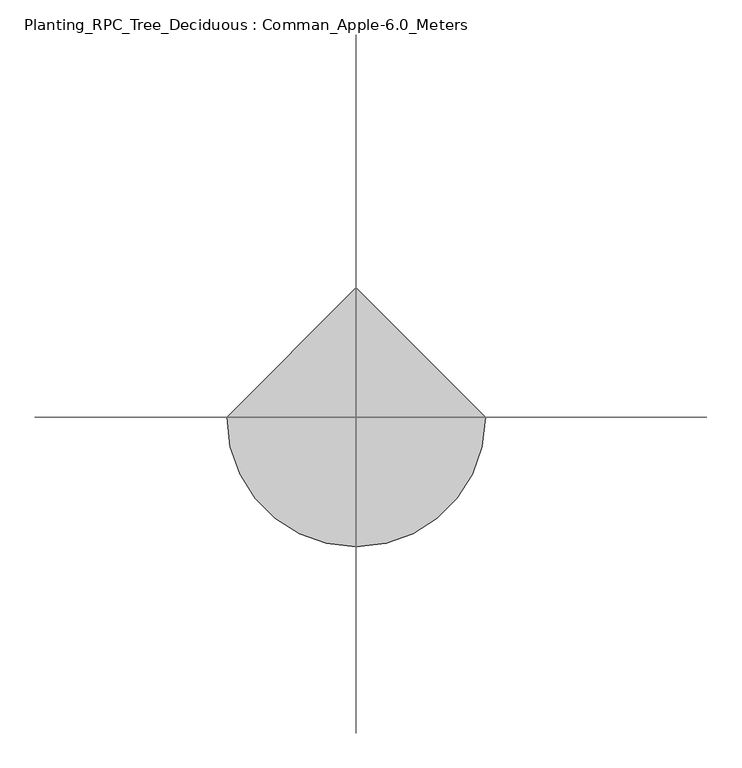
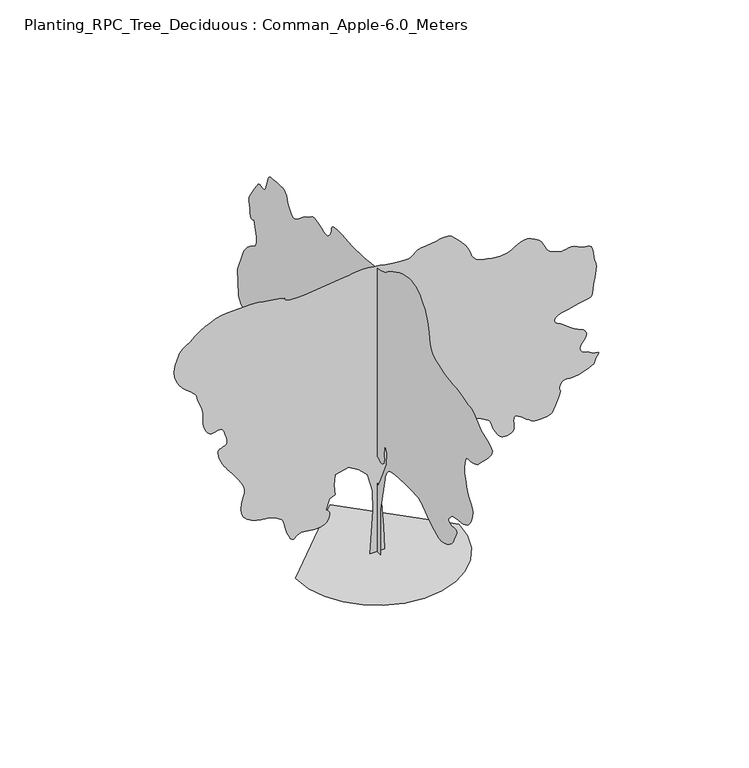
"""IFC4 building model written with IfcOpenShell, lengths in millimetres: geographic element geometry, Planting_RPC_Tree_Deciduous : Comman_Apple-6.0_Meters."""

from ifc_helpers import new_model, si_unit, origin, place, context, project, spatial, triangles, source, transform, mapped, element, save


def planting_rpc_tree_deciduous_comman_apple_6_0_meters_31fc5fb8(model_context):
    return source(origin(), model_context, "Body", "Tessellation", [
        triangles([(-6.51e-05, -105.0228319, 0.0074776), (-6.15e-05, 138.9131143, 0.0074703), (-4.84e-05, 99.8833291, 458.6078719), (-3.14e-05, 129.1556067, 1014.7807915), (-1.8e-05, 226.7299288, 1414.8361691), (-8.5e-06, 392.6053236, 1649.0138809), (-1.1e-06, 577.9979682, 1805.1340027), (2.6e-06, 753.6305981, 1844.161417), (3.5e-06, 948.7807503, 1775.8613708), (1.5e-06, 1007.3257959, 1678.2863674), (-4e-06, 890.2357046, 1551.4387321), (-8.4e-06, 929.2657351, 1385.5636826), (-1.44e-05, 1153.685903, 1073.3258371), (-1.47e-05, 1543.9838093, 868.4182137), (-8.5e-06, 2109.9142365, 790.3606236), (7.6e-06, 2451.4244957, 1161.1409712), (2.53e-05, 2802.702182, 1580.7112186), (3.2e-05, 3349.1028419, 1531.9237896), (3.84e-05, 3544.2528488, 1649.0138809), (4.53e-05, 3534.5028625, 1883.1915928), (4.5e-05, 3358.8778267, 1961.2516537), (4.95e-05, 3232.0277206, 2175.9142776), (5.43e-05, 3534.5028625, 2185.6718216), (5.98e-05, 4139.453437, 2068.584201), (6.19e-05, 4208.0283211, 2104.1717091), (6.39e-05, 4273.9283684, 2140.0142887), (6.59e-05, 4334.553447, 2176.3691917), (6.78e-05, 4387.2284294, 2213.4942513), (6.96e-05, 4429.328476, 2251.6417774), (7.12e-05, 4458.2034576, 2291.0693127), (7.26e-05, 4471.2035362, 2332.0343994), (8.79e-05, 4500.4784935, 2829.6522812), (9.79e-05, 4334.6034439, 3249.2275429), (9.86e-05, 4317.5036156, 3282.3275574), (9.94e-05, 4292.2284142, 3321.5527794), (0.0001002, 4260.1033401, 3364.7027618), (0.000101, 4222.5283081, 3409.5526405), (0.0001017, 4180.8532356, 3453.9028404), (0.0001023, 4136.4533295, 3495.527916), (0.0001027, 4090.6782166, 3532.2027122), (0.0001029, 4046.5782921, 3560.9279938), (0.0001029, 4006.7531067, 3582.8278198), (0.000103, 3971.8782005, 3601.8278229), (0.0001031, 3942.6282417, 3621.853054), (0.0001036, 3919.7031876, 3646.8529816), (0.0001043, 3903.7782875, 3680.7029503), (0.0001056, 3895.5282097, 3727.3530098), (0.0001072, 3894.4782738, 3782.2781456), (0.0001089, 3899.0532852, 3838.2282188), (0.0001108, 3908.3283005, 3895.0532387), (0.0001127, 3921.3530869, 3952.5282188), (0.0001147, 3937.2032822, 4010.528167), (0.0001167, 3954.9280724, 4068.8783844), (0.0001187, 3973.5780968, 4127.4033005), (0.0001184, 3998.5533165, 4107.2783661), (0.0001184, 4022.8532867, 4091.9534294), (0.0001185, 4045.7783409, 4086.1782005), (0.0001191, 4066.6532295, 4094.7532585), (0.0001202, 4084.8032845, 4122.4283134), (0.0001219, 4099.5532562, 4174.003363), (0.0001245, 4110.1781891, 4254.2534065), (0.000127, 4120.6784203, 4333.2285278), (0.0001287, 4132.0283089, 4385.4035408), (0.0001299, 4139.1284569, 4422.2036201), (0.0001309, 4136.8033081, 4455.0786484), (0.0001318, 4120.0034615, 4495.478508), (0.0001331, 4083.5533607, 4554.8286644), (0.0001348, 4022.3783157, 4644.5537109), (0.0001367, 3956.5782623, 4741.1289207), (0.0001382, 3906.9780922, 4815.003772), (0.0001392, 3869.5280525, 4868.5789902), (0.0001398, 3840.0781059, 4904.2041412), (0.0001401, 3814.5532104, 4924.3290756), (0.0001399, 3788.8780334, 4931.3042313), (0.0001393, 3758.9281174, 4927.5038818), (0.0001386, 3727.67799, 4918.0288788), (0.0001379, 3700.2029228, 4909.0788437), (0.0001374, 3675.45298, 4904.7291092), (0.0001372, 3652.4029335, 4909.0788437), (0.0001374, 3630.0528442, 4926.2289597), (0.000138, 3607.3527763, 4960.2792068), (0.0001393, 3583.2777924, 5015.329335), (0.0001409, 3562.2279144, 5079.6288986), (0.0001424, 3546.3027237, 5137.7544205), (0.0001437, 3531.0527824, 5188.4042358), (0.0001447, 3512.0527794, 5230.1540131), (0.0001452, 3484.8526955, 5261.6794144), (0.0001452, 3445.0278008, 5281.604361), (0.0001446, 3388.1277855, 5288.5295197), (0.0001436, 3319.3276245, 5291.5793335), (0.0001428, 3248.6275795, 5298.5544891), (0.000142, 3178.9774704, 5306.2040222), (0.0001411, 3113.2274139, 5311.3042923), (0.0001402, 3054.3025223, 5310.5793365), (0.0001392, 3005.1273262, 5300.8293503), (0.000138, 2968.5775223, 5278.7795334), (0.0001369, 2944.7272339, 5253.1543533), (0.0001361, 2929.602285, 5232.6294434), (0.0001354, 2919.9272942, 5214.0044174), (0.0001347, 2912.4774582, 5194.0044754), (0.0001338, 2904.0023941, 5169.4042328), (0.0001326, 2891.2523003, 5136.9288895), (0.000131, 2871.0023735, 5093.3792221), (0.0001292, 2844.6522377, 5045.379245), (0.0001275, 2815.5772682, 5003.1539154), (0.000126, 2783.4271957, 4968.9542587), (0.0001248, 2747.8773308, 4945.0039764), (0.0001238, 2708.5521149, 4933.504097), (0.0001233, 2665.1521477, 4936.7039017), (0.0001232, 2617.3021614, 4956.7788391), (0.0001234, 2569.6771614, 4988.2542435), (0.0001238, 2525.4769524, 5023.3038483), (0.0001243, 2482.1194244, 5060.7288895), (0.0001247, 2437.0595295, 5099.3538574), (0.0001252, 2387.7318718, 5138.0044052), (0.0001254, 2331.5768692, 5175.4294464), (0.0001255, 2266.0343582, 5210.4790512), (0.0001256, 2205.0142456, 5244.5542969), (0.0001259, 2159.0142918, 5277.6040237), (0.0001262, 2120.3541515, 5306.2290207), (0.0001262, 2081.3542065, 5327.0044968), (0.0001258, 2034.3291698, 5336.5044983), (0.0001247, 1971.6040741, 5331.3292328), (0.0001227, 1885.4940685, 5308.0544907), (0.0001205, 1797.391452, 5276.8540695), (0.0001188, 1730.2863911, 5251.9544266), (0.0001175, 1678.8813892, 5236.1042313), (0.0001168, 1637.8888332, 5232.02948), (0.0001166, 1602.0163136, 5242.4794235), (0.0001169, 1565.9737461, 5270.1544785), (0.0001177, 1524.4687214, 5317.8044769), (0.0001188, 1490.9861721, 5373.8045471), (0.0001201, 1475.2561729, 5423.9793915), (0.0001212, 1466.3511932, 5467.3296524), (0.0001221, 1453.3511147, 5502.8292297), (0.0001225, 1425.3286972, 5529.4543488), (0.0001222, 1371.366148, 5546.1794907), (0.000121, 1280.5334656, 5551.979718), (0.0001195, 1182.4759335, 5550.8792038), (0.0001183, 1108.9958982, 5547.8793869), (0.0001174, 1052.4133781, 5543.5296524), (0.0001165, 1005.0483187, 5538.3293884), (0.0001156, 959.2208107, 5532.7797272), (0.0001147, 907.2482563, 5527.4044739), (0.0001136, 841.4482029, 5522.7041794), (0.0001125, 772.3506037, 5519.7043625), (0.0001115, 711.6155754, 5518.9044113), (0.0001107, 653.2705175, 5520.154335), (0.0001099, 591.3404677, 5523.2797256), (0.000109, 519.8504273, 5528.1294296), (0.0001078, 432.8303392, 5534.5046219), (0.0001065, 324.3052774, 5542.2297318), (0.000105, 203.687658, 5552.8796631), (0.0001037, 86.9965703, 5567.6043457), (0.0001026, -21.8426915, 5585.7544006), (0.0001018, -118.9050968, 5606.6292892), (0.0001012, -200.2644113, 5629.5546341), (0.0001011, -261.9952181, 5653.8543137), (0.0001012, -300.1702499, 5678.8295334), (0.0001016, -342.4727732, 5713.0297714), (0.000102, -413.9603428, 5761.2297363), (0.0001023, -506.7854181, 5817.0798157), (0.0001024, -613.0930281, 5874.3298096), (0.0001023, -725.0330704, 5926.6045258), (0.0001019, -834.75319, 5967.6299286), (0.0001011, -934.4057556, 5991.07966), (0.0001, -1022.9033335, 5999.8047089), (9.88e-05, -1104.7484104, 6000.0046967), (9.74e-05, -1180.4459702, 5990.3047073), (9.57e-05, -1250.5110249, 5969.3298248), (9.38e-05, -1315.4560432, 5935.7295502), (9.14e-05, -1375.7936394, 5888.1545471), (8.87e-05, -1432.0336658, 5825.2049011), (8.63e-05, -1478.7161362, 5768.8048553), (8.48e-05, -1512.7687088, 5733.7546692), (8.36e-05, -1538.2837212, 5707.9295013), (8.25e-05, -1559.3638298, 5679.2045105), (8.09e-05, -1580.1012268, 5635.454274), (7.84e-05, -1604.5962433, 5564.5545319), (7.46e-05, -1636.941362, 5454.4042786), (7.05e-05, -1667.1512913, 5330.3292938), (6.7e-05, -1688.656374, 5223.97939), (6.39e-05, -1710.6739254, 5132.8541382), (6.11e-05, -1742.4214062, 5054.3292801), (5.83e-05, -1793.1164223, 4985.8788071), (5.53e-05, -1871.9714928, 4924.9540375), (5.19e-05, -1988.2065491, 4868.9789658), (4.87e-05, -2119.0091755, 4825.5040031), (4.62e-05, -2237.6917568, 4799.6038399), (4.41e-05, -2347.6668755, 4784.9788605), (4.22e-05, -2452.3543808, 4775.3288681), (4.04e-05, -2555.1521759, 4764.2789612), (3.83e-05, -2659.5022018, 4745.5539413), (3.57e-05, -2768.8022163, 4712.8539024), (3.33e-05, -2866.4523605, 4683.5786545), (3.19e-05, -2939.5522591, 4672.2287659), (3.09e-05, -2996.927536, 4668.05373), (2.99e-05, -3047.4773575, 4660.2786232), (2.85e-05, -3100.0776352, 4638.1788094), (2.61e-05, -3163.6025368, 4590.9787834), (2.24e-05, -3246.9276833, 4507.9536186), (1.83e-05, -3354.9527756, 4422.0536293), (1.48e-05, -3474.4277504, 4364.5036537), (1.18e-05, -3586.9278603, 4321.8033531), (9.3e-06, -3673.9780701, 4280.47855), (7e-06, -3717.153051, 4227.0283241), (5e-06, -3698.0280556, 4147.9782074), (2.9e-06, -3598.1780457, 4029.8281517), (1.1e-06, -3473.4528099, 3906.2781349), (-3e-07, -3385.2276718, 3815.6781418), (-1.3e-06, -3323.4776619, 3751.5279877), (-1.9e-06, -3278.1025246, 3707.3530678), (-2.2e-06, -3239.0275841, 3676.6529068), (-2.3e-06, -3196.2275803, 3652.9528999), (-2.1e-06, -3139.5775497, 3629.777861), (-1.7e-06, -3075.1774109, 3613.37799), (-9e-07, -3016.2275208, 3608.6029907), (-2e-07, -2963.4272552, 3606.7278145), (2e-07, -2917.4774437, 3599.0529922), (2e-07, -2879.0024666, 3576.8528938), (-7e-07, -2848.7272797, 3531.452758), (-2.7e-06, -2827.3524216, 3454.1278267), (-5.1e-06, -2815.7522575, 3369.9277336), (-7e-06, -2813.352404, 3305.0276253), (-8.6e-06, -2818.6523712, 3252.4026398), (-1.02e-05, -2830.0772552, 3205.052623), (-1.19e-05, -2846.1274384, 3156.0024193), (-1.39e-05, -2865.2274353, 3098.2524559), (-1.64e-05, -2885.9023361, 3024.8025787), (-1.92e-05, -2914.627327, 2946.6774055), (-2.18e-05, -2954.4525124, 2877.5772629), (-2.43e-05, -2998.5524368, 2814.6273262), (-2.67e-05, -3040.0775185, 2754.9021927), (-2.9e-05, -3072.2275909, 2695.5270378), (-3.11e-05, -3088.152491, 2633.6020386), (-3.3e-05, -3081.0526337, 2566.2020828), (-3.46e-05, -3060.4274391, 2500.277037), (-3.6e-05, -3039.102578, 2443.7194427), (-3.71e-05, -3015.2525803, 2395.18694), (-3.79e-05, -2986.9272743, 2353.3118797), (-3.85e-05, -2952.3273514, 2316.7293743), (-3.88e-05, -2909.5023491, 2284.0717747), (-3.89e-05, -2856.6273788, 2253.9743385), (-3.87e-05, -2791.7272705, 2230.5618141), (-3.8e-05, -2717.452153, 2216.0268002), (-3.71e-05, -2638.7520149, 2206.0967377), (-3.62e-05, -2560.5271385, 2196.5117123), (-3.56e-05, -2487.799601, 2182.9993103), (-3.53e-05, -2425.47201, 2161.2942398), (-3.56e-05, -2378.5043827, 2127.129174), (-3.62e-05, -2345.7043499, 2089.8041267), (-3.68e-05, -2322.8044395, 2060.3341232), (-3.73e-05, -2310.1443111, 2037.0066227), (-3.78e-05, -2308.0692924, 2018.1191128), (-3.84e-05, -2316.9168629, 2001.9616688), (-3.92e-05, -2337.0294434, 1986.8265461), (-4.01e-05, -2368.7469841, 1971.0090523), (-4.1e-05, -2411.2470062, 1962.5040482), (-4.16e-05, -2459.0394379, 1965.0915356), (-4.21e-05, -2505.4770103, 1970.754126), (-4.27e-05, -2543.876992, 1971.4641117), (-4.34e-05, -2567.6019974, 1959.2041042), (-4.44e-05, -2569.9771431, 1925.949012), (-4.59e-05, -2544.3769615, 1863.6765049), (-4.75e-05, -2509.7520401, 1792.5014889), (-4.89e-05, -2484.8695473, 1735.1513557), (-4.99e-05, -2462.7095627, 1687.5312973), (-5.08e-05, -2436.2819607, 1645.5438892), (-5.14e-05, -2398.5894939, 1605.0912712), (-5.19e-05, -2342.631863, 1562.0787804), (-5.22e-05, -2261.4142914, 1512.4087017), (-5.2e-05, -2169.1316975, 1473.3237328), (-5.1e-05, -2083.5066914, 1461.3762062), (-4.95e-05, -2002.8290577, 1471.4462311), (-4.76e-05, -1925.3965748, 1498.4137711), (-4.53e-05, -1849.4990273, 1537.1587898), (-4.28e-05, -1773.4289612, 1582.5612511), (-4.02e-05, -1695.4838642, 1629.498793), (-3.77e-05, -1622.0063725, 1676.8063705), (-3.54e-05, -1558.0838207, 1724.7964645), (-3.31e-05, -1500.136195, 1770.5689613), (-3.11e-05, -1444.578685, 1811.2214218), (-2.93e-05, -1387.8261898, 1843.8489361), (-2.77e-05, -1326.2960793, 1865.5564774), (-2.64e-05, -1256.4010723, 1873.4340488), (-2.5e-05, -1159.1384045, 1874.2890839), (-2.3e-05, -1027.910804, 1875.4840691), (-2.07e-05, -877.7382116, 1874.971455), (-1.86e-05, -723.6380974, 1870.7039829), (-1.67e-05, -580.6329818, 1860.6339581), (-1.55e-05, -463.7428782, 1842.7115055), (-1.52e-05, -387.9878002, 1814.8914013), (-1.57e-05, -343.2127716, 1776.8839828), (-1.66e-05, -308.1652379, 1730.6863667), (-1.77e-05, -281.2252217, 1677.6614056), (-1.92e-05, -260.7727092, 1619.1738419), (-2.08e-05, -245.1829449, 1556.5887085), (-2.26e-05, -232.8366963, 1491.2736546), (-2.44e-05, -222.1121874, 1424.593713), (-3.85e-05, -114.7803395, 897.6907001), (-2.01e-05, -26.9632729, 1297.7460777), (-1.3e-05, -173.3248856, 1609.9838505), (-6.5e-06, -300.1727388, 1892.9489914), (2e-07, -319.6852469, 2127.129174), (4.7e-06, -251.3852008, 2244.2167946), (-4e-07, -222.1119331, 2058.8266571), (-1.7e-06, -228.0859325, 2017.1791992), (-3e-06, -232.2679447, 1976.5565334), (-4.1e-06, -232.865183, 1937.9815624), (-5.1e-06, -228.0859325, 1902.4790783), (-5.9e-06, -216.1379336, 1871.0740185), (-6.4e-06, -195.2293988, 1844.788995), (-6.5e-06, -163.5673779, 1824.6489452), (-6.1e-06, -127.1833524, 1819.4714996), (-5.2e-06, -93.5303284, 1831.0190506), (-4.2e-06, -62.949051, 1849.7389835), (-3.3e-06, -35.7820297, 1866.0664753), (-2.9e-06, -12.3698845, 1870.4490566), (-3.1e-06, 6.9458055, 1853.3239391), (-4.3e-06, 21.8237678, 1805.1340027), (-6.1e-06, 32.3777771, 1741.0688725), (-7.7e-06, 39.3472803, 1682.1263947), (-9.3e-06, 43.330036, 1627.4512436), (-1.08e-05, 44.9230347, 1576.1888203), (-1.22e-05, 44.724037, 1527.4862698), (-1.37e-05, 43.330036, 1480.4911732), (-1.51e-05, 41.3385332, 1434.3511116), (137.391859, 0.0003253, 0.0), (-133.3141101, 0.0003334, 0.0), (-73.1573078, 0.0002372, 832.1731876), (-83.1833128, 0.0002433, 1223.1935062), (-183.4456522, 0.0001982, 1574.1087147), (-333.8377625, 0.0002049, 1724.5014244), (-534.3604428, 0.0002126, 1844.8164642), (-785.015601, 0.0002192, 1784.6589443), (-805.0681561, 0.0002168, 1584.1363003), (-785.015601, 0.0002134, 1393.6386257), (-885.278231, 0.0002156, 1343.5060753), (-955.4607931, 0.0002149, 1153.0084007), (-936.3432827, 0.0002675, 1139.8859459), (-918.5407356, 0.0002668, 1125.3558735), (-903.3707314, 0.0002661, 1108.0234285), (-892.1456898, 0.0002654, 1086.4808481), (-886.1831903, 0.0002648, 1059.3258196), (-886.7981964, 0.0002643, 1025.1533415), (-895.3032005, 0.0002639, 982.5658247), (-913.9532249, 0.0002639, 940.0632591), (-942.5982788, 0.0002642, 906.5057144), (-978.963283, 0.0002649, 881.018244), (-1020.7633478, 0.0002659, 862.7181982), (-1065.71838, 0.0002671, 850.7331739), (-1111.553373, 0.0002683, 844.1856812), (-1155.9834372, 0.0002696, 842.1981571), (-1199.4784567, 0.000271, 844.8881819), (-1243.6759769, 0.0002724, 851.4356747), (-1288.0485592, 0.0002738, 859.5631582), (-1332.0685467, 0.0002752, 866.9856703), (-1375.2135876, 0.0002766, 871.4282043), (-1416.9560978, 0.0002778, 870.610667), (-1456.7686386, 0.0002789, 862.2507122), (-1490.9986713, 0.0002796, 844.3906832), (-1518.2137253, 0.0002801, 821.2681847), (-1541.2187164, 0.0002805, 799.9006662), (-1562.8187061, 0.0002809, 787.3031067), (-1585.8238426, 0.0002817, 790.4881594), (-1613.0387512, 0.0002829, 816.475672), (-1647.2663132, 0.0002313, 872.2782251), (-1679.7413658, 0.0002334, 944.3882858), (-1702.0463997, 0.0002351, 1013.34585), (-1717.508828, 0.0002365, 1077.2133905), (-1729.4639122, 0.0002377, 1134.0684231), (-1741.2438618, 0.0002387, 1181.9784348), (-1756.1814674, 0.0002397, 1219.0134562), (-1777.6064678, 0.0002407, 1243.2460613), (-1804.2939377, 0.0002418, 1262.5659576), (-1833.963929, 0.000243, 1284.8709915), (-1868.368951, 0.0002444, 1308.2261066), (-1909.2639839, 0.000246, 1330.7035137), (-1958.3990662, 0.0002477, 1350.3761501), (-2017.5341194, 0.0002497, 1365.3136105), (-2088.4191822, 0.0002519, 1373.5860706), (-2170.7616852, 0.0002011, 1382.5010788), (-2258.5417923, 0.000204, 1401.9387005), (-2344.9193687, 0.0002071, 1433.8312305), (-2423.054425, 0.0002101, 1480.1036968), (-2486.1046463, 0.0002129, 1542.6862141), (-2527.2271362, 0.0002153, 1623.5087517), (-2539.6019623, 0.0002172, 1724.5014244), (-2528.5270569, 0.0002183, 1822.2489464), (-2508.6771057, 0.0002189, 1897.5490013), (-2487.2420769, 0.0002192, 1958.6416386), (-2471.4293793, 0.0001661, 2013.7690876), (-2468.4170631, 0.0001669, 2071.1791008), (-2485.3994568, 0.0001684, 2139.1117275), (-2529.5769928, 0.000171, 2225.8093426), (-2588.3771828, 0.0001741, 2318.6769299), (-2644.0272743, 0.000177, 2400.3194756), (-2695.8273102, 0.0001796, 2471.7869156), (-2743.0773331, 0.000182, 2534.1270058), (-2785.0523872, 0.0001306, 2588.4271797), (-2821.0522247, 0.0001324, 2635.6772026), (-2850.4021774, 0.0001339, 2676.977298), (-2878.5522034, 0.0001354, 2723.8270546), (-2908.6274025, 0.0001372, 2782.7522369), (-2936.4274498, 0.000139, 2847.4523575), (-2957.7523109, 0.0001406, 2911.6522179), (-2968.352536, 0.0001418, 2969.0024963), (-2964.0525078, 0.0001423, 3013.2024147), (-2940.6524826, 0.000142, 3037.927359), (-2905.0023331, 0.0001411, 3050.052491), (-2869.2021927, 0.0001402, 3062.5526001), (-2836.7274307, 0.0001395, 3078.1775185), (-2811.1022507, 0.000139, 3099.7773628), (-2795.8023125, 0.000139, 3130.1525436), (-2794.3773994, 0.0001396, 3172.1025993), (-2810.3022995, 0.0001409, 3228.4276497), (-2831.7271545, 8.9e-05, 3286.3526024), (-2846.6774048, 9.02e-05, 3332.2027107), (-2858.4522675, 9.1e-05, 3367.3276016), (-2870.4024101, 9.18e-05, 3393.1777679), (-2885.8523392, 9.25e-05, 3411.1278351), (-2908.17743, 9.33e-05, 3422.5777176), (-2940.6524826, 9.44e-05, 3428.9529099), (-2978.7524826, 9.55e-05, 3427.0527351), (-3016.0025345, 9.65e-05, 3417.4277412), (-3052.7023293, 9.74e-05, 3407.1277885), (-3089.2524239, 9.85e-05, 3403.1027435), (-3125.9775078, 9.97e-05, 3412.4277557), (-3163.2025612, 0.0001012, 3442.1026886), (-3201.3275597, 0.0001032, 3499.1276962), (-3229.5025841, 0.0001051, 3569.6277534), (-3241.3777313, 0.0001065, 3637.1529922), (-3243.9525742, 0.0001076, 3704.8529297), (-3244.2275574, 0.0001086, 3775.9029533), (-3249.2525414, 5.65e-05, 3853.4031647), (-3266.0276802, 5.83e-05, 3940.5780762), (-3301.5775452, 6.09e-05, 4040.5533691), (-3337.877655, 6.33e-05, 4130.928376), (-3357.5276184, 6.48e-05, 4192.7283829), (-3368.4028267, 6.58e-05, 4234.1784691), (-3378.4027977, 6.65e-05, 4263.5284218), (-3395.4276306, 6.74e-05, 4289.0033203), (-3427.3277184, 6.88e-05, 4318.8785316), (-3482.0528664, 7.1e-05, 4361.3785538), (-3552.8529053, 2.06e-05, 4417.8785934), (-3623.6529442, 2.37e-05, 4484.3786041), (-3688.3030678, 2.68e-05, 4561.0535751), (-3740.6780685, 2.96e-05, 4648.0787865), (-3774.6530296, 3.21e-05, 4745.6289368), (-3784.0780357, 3.4e-05, 4853.8540169), (-3762.7781731, 3.51e-05, 4972.9790131), (-3729.8781464, -1.77e-05, 5076.7040771), (-3704.502951, -1.74e-05, 5145.8539261), (-3680.7029503, -1.74e-05, 5191.3290573), (-3652.5279259, -1.78e-05, 5224.0043884), (-3614.0029518, -1.85e-05, 5254.7792542), (-3559.1778099, -1.95e-05, 5294.454158), (-3482.0528664, -2.09e-05, 5353.9795944), (-3391.1775993, -2.26e-05, 5424.8793365), (-3298.9027084, -2.44e-05, 5490.3794083), (-3205.0276245, -2.63e-05, 5548.6543396), (-3109.4276459, -2.84e-05, 5598.0042343), (-3011.8774956, -3.07e-05, 5636.6297836), (-2912.2274734, -3.33e-05, 5662.8293472), (-2810.3022995, -3.62e-05, 5674.8047791), (-2339.0719059, -5.01e-05, 5684.8297485), (-2273.3618179, -5.21e-05, 5682.2043274), (-2197.6542297, -5.44e-05, 5674.854776), (-2113.614156, -3.7e-06, 5663.5293045), (-2022.9116982, -6.6e-06, 5649.0546066), (-1927.2115803, -9.7e-06, 5632.2294708), (-1828.1764915, -1.3e-05, 5613.8044327), (-1727.4763882, -1.63e-05, 5594.6044418), (-1724.3188774, -1.66e-05, 5575.4544479), (-1715.1114452, -1.72e-05, 5557.4543839), (-1693.8014088, -1.8e-05, 5541.7297623), (-1654.3413174, -1.94e-05, 5529.4293503), (-1590.6763081, -2.14e-05, 5521.6792419), (-1496.7561687, -2.42e-05, 5519.6293671), (-1366.5335941, -2.81e-05, 5524.4296555), (-604.5454757, -4.94e-05, 5614.6543808), (-529.8304141, -5.15e-05, 5621.554541), (-464.7628741, 1e-07, 5631.7794983), (-403.0278342, -1.6e-06, 5642.554422), (-338.3102729, -3.4e-06, 5651.0294861), (-264.297712, -5.6e-06, 5654.4042801), (-174.6758932, -8.3e-06, 5649.9045547), (-63.1313028, -1.19e-05, 5634.7043198), (53.8502923, -1.57e-05, 5614.4793915), (156.9766284, -1.9e-05, 5596.879303), (248.3524462, -2.19e-05, 5582.1046234), (330.0827591, -2.45e-05, 5570.2797638), (404.2703093, -2.69e-05, 5561.6297104), (473.0203643, -2.9e-05, 5556.304454), (538.4379192, -3.1e-05, 5554.5045639), (593.7429737, -3.25e-05, 5562.8296371), (635.895488, -3.35e-05, 5584.3044891), (672.6080727, -3.41e-05, 5613.6794403), (711.6030762, -3.48e-05, 5645.7048111), (760.5931091, -3.58e-05, 5675.0797623), (827.2981945, -3.75e-05, 5696.5546143), (919.4332684, -4.01e-05, 5704.904686), (1019.3733164, -4.3e-05, 5711.6048584), (1106.3358862, -4.54e-05, 5726.7545151), (1183.3009558, -4.74e-05, 5742.7796997), (1253.2485031, -4.94e-05, 5752.1297104), (1319.1661366, -5.14e-05, 5747.279425), (1384.0286018, -5.37e-05, 5720.6798859), (1450.8211819, -3.2e-06, 5664.7798096), (1514.7787605, -6.1e-06, 5597.4042709), (1569.6162563, -8.6e-06, 5539.5043167), (1616.0337719, -1.07e-05, 5488.254538), (1654.7363514, -1.26e-05, 5440.8795227), (1686.421336, -1.42e-05, 5394.5544434), (1711.7939152, -1.57e-05, 5346.4544724), (1731.5539009, -1.7e-05, 5293.8291962), (1749.3263626, -1.84e-05, 5241.0045135), (1770.606459, -1.97e-05, 5194.1544662), (1798.9013889, -2.12e-05, 5153.0790665), (1837.7189323, 3.06e-05, 5117.6039063), (1890.5690495, 2.85e-05, 5087.6039932), (1960.9566135, 2.61e-05, 5062.8293427), (2052.3917301, 2.3e-05, 5043.1537994), (2147.2741653, 2e-05, 5028.9540848), (2227.0742363, 1.75e-05, 5020.3540283), (2293.8969017, 1.55e-05, 5016.8542419), (2349.8443588, 1.38e-05, 5017.9041779), (2397.0244732, 1.25e-05, 5023.0038666), (2437.5369713, 1.14e-05, 5031.5789246), (2473.4920441, 1.05e-05, 5043.1537994), (2512.0269012, 9.7e-06, 5063.479303), (2558.2519867, 8.7e-06, 5093.9791855), (2611.3522339, 7.6e-06, 5127.6038773), (2670.3771194, 6.3e-06, 5157.4043839), (2734.5272736, 4.7e-06, 5176.304393), (2802.8521729, 2.7e-06, 5177.3293304), (2874.527449, 2e-07, 5153.4540436), (2937.3023964, -2.2e-06, 5120.2293274), (2982.5275429, -3.9e-06, 5095.0541199), (3014.7523201, -5.2e-06, 5073.7292587), (3038.5773193, -6.2e-06, 5052.0788361), (3058.5525536, -7.2e-06, 5025.854274), (3079.2024559, -8.3e-06, 4990.8790833), (3105.1276176, -9.8e-06, 4942.9041046), (3132.7273865, 4.2e-05, 4892.8036743), (3157.7026062, 4.07e-05, 4852.7037964), (3183.5274834, 3.94e-05, 4820.3040298), (3213.7526733, 3.81e-05, 4793.3539307), (3251.8776718, 3.66e-05, 4769.5539299), (3301.4025558, 3.48e-05, 4746.6538742), (3365.8276932, 3.25e-05, 4722.3289055), (3431.1277771, 3.03e-05, 4707.5039383), (3484.3277275, 2.88e-05, 4709.3538254), (3530.502816, 2.76e-05, 4719.9537598), (3574.753022, 2.64e-05, 4731.4539299), (3622.1780342, 2.51e-05, 4735.9289474), (3677.8278351, 2.33e-05, 4725.4787132), (3746.8029854, 2.07e-05, 4692.2537064), (3818.1279922, 1.81e-05, 4658.4537346), (3877.8781242, 1.61e-05, 4644.1287369), (3926.7530479, 1.45e-05, 4638.053817), (3965.453302, 1.32e-05, 4629.003788), (3994.7032608, 1.2e-05, 4605.7287552), (4015.1531754, 6.41e-05, 4557.0288208), (4027.5532906, 6.24e-05, 4471.6785072), (4039.2031609, 6.08e-05, 4384.4785973), (4054.5533867, 5.95e-05, 4327.8035683), (4069.9033218, 5.84e-05, 4286.7284592), (4081.5781906, 5.75e-05, 4246.3533073), (4085.8532204, 5.65e-05, 4191.7784409), (4079.1033417, 5.55e-05, 4108.1033157), (4057.628199, 5.42e-05, 3980.3782631), (4035.5283852, 0.0001063, 3847.1779633), (4024.4781876, 0.0001052, 3752.0279572), (4017.103347, 0.0001045, 3687.578112), (4006.0531494, 0.0001042, 3646.453006), (3983.9533356, 0.0001045, 3621.2777985), (3943.4531914, 0.0001054, 3604.7279366), (3877.1531685, 0.0001072, 3589.3780014), (3783.9280449, 0.0001097, 3571.4279343), (3675.2779907, 0.0001126, 3551.3779953), (3562.7778809, 0.0001156, 3528.3279488), (3457.9778824, 0.0001183, 3501.452845), (3372.4778687, 0.0001204, 3469.8277405), (3317.8527145, 0.0001215, 3432.5776886), (3305.6525871, 0.0001212, 3388.8527412), (3318.4276794, 0.0001203, 3351.9776665), (3332.9526649, 0.0001195, 3330.9027901), (3352.2276512, 0.0001188, 3318.0777008), (3379.2027489, 0.0001178, 3305.9525688), (3416.8777748, 0.0001164, 3286.9775642), (3468.2528366, 0.0001143, 3253.627565), (3536.2527557, 0.0001115, 3198.3524506), (3611.5028137, 0.0001084, 3139.7525391), (3681.477903, 0.0001057, 3097.8024834), (3744.6281181, 0.0001033, 3067.0776146), (3799.3529755, 0.0001547, 3042.1273933), (3844.053154, 0.000153, 3017.5524399), (3877.2031654, 0.0001516, 2987.877507), (3897.2031075, 0.0001504, 2947.702343), (3897.9280632, 0.0001497, 2900.4773186), (3879.7280113, 0.0001495, 2853.6272713), (3850.6530418, 0.0001497, 2807.4771812), (3818.7529541, 0.00015, 2762.3773178), (3792.1281258, 0.0001501, 2718.6770782), (3778.8280655, 0.0001499, 2676.7270226), (3786.9281525, 0.0001491, 2636.8771294), (3809.6282204, 0.0001479, 2605.4770111), (3834.8031372, 0.0001469, 2585.8520462), (3862.4281952, 0.0001459, 2573.7522034), (3892.5031036, 0.0001448, 2564.9771576), (3925.0281532, 0.0001437, 2555.3271652), (3960.0283424, 0.0001425, 2540.6021919), (3997.4780914, 0.000141, 2516.5769142), (4036.1783455, 0.0001395, 2494.674472), (4072.603157, 0.0001383, 2485.0596519), (4103.2283226, 0.0001373, 2481.5796318), (4124.5534744, 0.0001366, 2478.1019371), (4133.1032433, 0.0001362, 2468.4845009), (4125.3284271, 0.0001895, 2446.5919418), (4097.7283676, 0.0001897, 2406.2819023), (4070.2033035, 0.0001899, 2361.9969601), (4057.9281807, 0.0001898, 2329.461882), (4050.3783508, 0.0001896, 2304.4693668), (4037.0532921, 0.0001897, 2282.8093517), (4007.4033577, 0.0001903, 2260.27439), (3950.9283165, 0.0001915, 2232.649332), (3857.1032295, 0.0001938, 2195.731818), (3751.1030136, 0.0001965, 2165.9741867), (3663.5278358, 0.000199, 2156.5616798), (3591.9278458, 0.0002011, 2158.3742146), (3533.8029053, 0.0002029, 2162.291708), (3486.7528702, 0.0002043, 2159.1942226), (3448.2778931, 0.0002051, 2139.9592049), (3415.9528313, 0.0002054, 2095.4691879), (3396.9028313, 0.0002053, 2048.9641777), (3394.8526657, 0.000205, 2022.9766651), (3402.2777939, 0.0002045, 2007.3391022), (3411.6278046, 0.000204, 1991.8766739), (3415.3778664, 0.0002035, 1966.4166), (3405.9528603, 0.0002031, 1920.7865364), (3375.8526627, 0.0002029, 1844.8164642), (3339.8028282, 0.0002027, 1759.2289558), (3313.4026955, 0.0002024, 1690.476321), (3290.3526489, 0.0002023, 1636.9838013), (3264.3024948, 0.0002025, 1597.1712605), (3228.9526176, 0.0002032, 1569.4613239), (3178.0025299, 0.0002044, 1552.2737103), (3105.1276176, 0.0002065, 1544.0311901), (3032.1274223, 0.0002086, 1540.6111954), (2980.1523972, 0.0002101, 1539.996262), (2942.0273987, 0.0002113, 1543.7687061), (2910.5772835, 0.0002124, 1553.5012516), (2878.6022003, 0.0002136, 1570.7762146), (2838.902298, 0.0002152, 1597.1712605), (2784.3021423, 0.0002174, 1634.2663799), (2725.2272598, 0.0002198, 1675.6263554), (2676.327047, 0.0002218, 1712.2539162), (2636.7271385, 0.0002234, 1741.8638821), (2605.5270081, 0.0002246, 1762.1813919), (2581.8769981, 0.0002254, 1770.9214108), (2564.9021622, 0.0002259, 1765.8039906), (2553.7019737, 0.0002259, 1744.5539795), (2547.3770691, 0.0002257, 1717.2514309), (2544.9269279, 0.0002254, 1694.3364052), (2545.2771973, 0.0002251, 1674.0488354), (2547.3770691, 0.0002247, 1654.6388283), (2550.2021873, 0.0002244, 1634.3538746), (2552.6520378, 0.0002239, 1611.4362328), (2553.7019737, 0.0002235, 1584.1363003), (2552.2770607, 0.0002231, 1554.2312943), (2547.1520828, 0.0002228, 1525.3811657), (2537.1271133, 0.0002227, 1498.6361412), (2520.9519379, 0.0002229, 1475.0461567), (2497.4295364, 0.0002233, 1455.666235), (2465.3044624, 0.000224, 1441.5461666), (2423.3594936, 0.0002251, 1433.7435905), (2380.6244568, 0.0002264, 1432.0761051), (2345.4293667, 0.0002275, 1436.3736626), (2315.4968914, 0.0002286, 1447.6861988), (2288.5467922, 0.0002297, 1467.0661205), (2262.2967957, 0.0002309, 1495.5662704), (2234.4692791, 0.0002323, 1534.2387646), (2202.7842945, 0.000234, 1584.1363003), (2173.4642818, 0.0002356, 1638.6213467), (2152.3892601, 0.0001837, 1689.7763638), (2136.7516972, 0.0001848, 1736.7214634), (2123.7442062, 0.0001858, 1778.5789375), (2110.561726, 0.0001868, 1814.4739849), (2094.3967243, 0.0001877, 1843.5290428), (2072.4441399, 0.0001886, 1864.8690193), (2041.9866966, 0.0001898, 1883.516573), (2003.1091278, 0.0001913, 1904.796524), (1957.2165802, 0.000193, 1928.2690739), (1905.7115845, 0.0001949, 1953.4966038), (1849.996526, 0.000197, 1980.0365536), (1791.4764061, 0.0001991, 2007.4566822), (1731.5539009, 0.0002013, 2035.3141388), (1390.663662, 0.0002115, 2035.3141388), (1200.1659874, 0.0002139, 1814.7364689), (1195.6959841, 0.0002136, 1784.6589443), (1190.1709579, 0.0002133, 1754.578949), (1182.5409731, 0.0002131, 1724.5014244), (1171.7559483, 0.0002129, 1694.4238998), (1156.7584625, 0.0002129, 1664.3439045), (1136.5034489, 0.0002131, 1634.2663799), (1109.9308702, 0.0002134, 1604.1888554), (1086.2834038, 0.0002138, 1578.7562508), (1071.7558748, 0.0002139, 1561.5687824), (1060.7358353, 0.0002141, 1551.0463142), (1047.610837, 0.0002144, 1545.6087101), (1026.7683592, 0.000215, 1543.6787407), (992.5982792, 0.000216, 1543.6787407), (939.4857508, 0.0002176, 1544.0311901), (873.0156801, 0.0002196, 1546.8661915), (804.2656614, 0.0002218, 1554.4362236), (735.8656214, 0.000224, 1565.3387558), (670.4455593, 0.0002262, 1578.1712574), (610.6404888, 0.0002281, 1591.5313431), (559.0754677, 0.0002299, 1604.0112499), (518.3879076, 0.0002312, 1614.2138248), (483.4279049, 0.0002324, 1624.5613037), (447.4153502, 0.0002337, 1638.0662933), (410.5253417, 0.000235, 1654.201355), (372.9353033, 0.0002364, 1672.4413754), (334.8177535, 0.0001845, 1692.2589157), (296.3502432, 0.0001859, 1713.1313335), (257.7052002, 0.0001874, 1734.5288647), (77.2350658, 0.0002405, 1353.5336609), (67.2090562, 0.0002365, 1062.7733562), (117.339849, 0.0002792, 451.1778749), (-1522.7162121, 1.1e-06, 0.0098235), (-1482.4612564, -348.9052657, 0.0098339), (-1367.8136032, -669.3205553, 0.0098435), (-1187.9534334, -952.0632534, 0.0098519), (-952.0632534, -1187.9534334, 0.0098589), (-669.3205553, -1367.8136032, 0.0098643), (-348.9052657, -1482.4612564, 0.0098677), (6.66e-05, -1522.7162121, 0.0098689), (348.9052657, -1482.4612564, 0.0098677), (669.3205553, -1367.8136032, 0.0098643), (952.0632534, -1187.9534334, 0.0098589), (1187.9534334, -952.0632534, 0.0098519), (1367.8136032, -669.3205553, 0.0098435), (1482.4612564, -348.9052657, 0.0098339), (1522.7162121, 0.0001238, 0.0098235), (-0.0001997, 1522.7162121, 0.0097782)], [[300, 1, 301], [299, 300, 301], [299, 301, 302], [298, 299, 302], [297, 298, 302], [296, 297, 302], [296, 302, 303], [295, 296, 303], [294, 295, 303], [293, 294, 303], [292, 293, 303], [1, 2, 3], [301, 1, 3], [301, 3, 4], [301, 4, 5], [327, 301, 5], [326, 327, 5], [326, 5, 6], [325, 326, 6], [324, 325, 6], [323, 324, 6], [322, 323, 6], [321, 322, 6], [320, 321, 6], [19, 20, 21], [18, 19, 21], [17, 18, 21], [17, 21, 22], [320, 6, 7], [319, 320, 7], [291, 292, 303], [291, 303, 304], [290, 291, 304], [261, 262, 263], [260, 261, 263], [260, 263, 264], [259, 260, 264], [259, 264, 265], [258, 259, 265], [10, 11, 12], [14, 15, 16], [258, 265, 266], [257, 258, 266], [205, 206, 207], [204, 205, 207], [204, 207, 208], [203, 204, 208], [203, 208, 209], [202, 203, 209], [202, 209, 210], [257, 266, 267], [10, 12, 13], [257, 267, 268], [257, 268, 269], [256, 257, 269], [256, 269, 270], [256, 270, 271], [255, 256, 271], [255, 271, 272], [255, 272, 273], [255, 273, 274], [255, 274, 275], [255, 275, 276], [255, 276, 277], [254, 255, 277], [254, 277, 278], [254, 278, 279], [254, 279, 280], [253, 254, 280], [253, 280, 281], [253, 281, 282], [289, 290, 304], [10, 13, 14], [10, 14, 16], [10, 16, 17], [10, 17, 22], [9, 10, 22], [201, 202, 210], [201, 210, 211], [201, 211, 212], [201, 212, 213], [201, 213, 214], [201, 214, 215], [201, 215, 216], [201, 216, 217], [201, 217, 218], [201, 218, 219], [200, 201, 219], [199, 200, 219], [198, 199, 219], [197, 198, 219], [196, 197, 219], [195, 196, 219], [194, 195, 219], [194, 219, 220], [193, 194, 220], [192, 193, 220], [191, 192, 220], [190, 191, 220], [189, 190, 220], [189, 220, 221], [188, 189, 221], [252, 253, 282], [252, 282, 283], [188, 221, 222], [187, 188, 222], [251, 252, 283], [187, 222, 223], [23, 24, 25], [318, 319, 7], [56, 57, 58], [56, 58, 59], [55, 56, 59], [55, 59, 60], [54, 55, 60], [54, 60, 61], [54, 61, 62], [23, 25, 26], [186, 187, 223], [23, 26, 27], [23, 27, 28], [23, 28, 29], [23, 29, 30], [23, 30, 31], [23, 31, 32], [23, 32, 33], [23, 33, 34], [23, 34, 35], [23, 35, 36], [23, 36, 37], [23, 37, 38], [23, 38, 39], [23, 39, 40], [23, 40, 41], [23, 41, 42], [23, 42, 43], [23, 43, 44], [22, 23, 44], [22, 44, 45], [9, 22, 45], [9, 45, 46], [9, 46, 47], [9, 47, 48], [8, 9, 48], [8, 48, 49], [8, 49, 50], [8, 50, 51], [8, 51, 52], [8, 52, 53], [8, 53, 54], [250, 251, 283], [250, 283, 284], [288, 289, 304], [288, 304, 305], [186, 223, 224], [287, 288, 305], [313, 314, 315], [312, 313, 315], [311, 312, 315], [310, 311, 315], [310, 315, 316], [309, 310, 316], [308, 309, 316], [308, 316, 317], [307, 308, 317], [306, 307, 317], [306, 317, 318], [305, 306, 318], [305, 318, 7], [305, 7, 8], [305, 8, 54], [305, 54, 62], [305, 62, 63], [305, 63, 64], [305, 64, 65], [305, 65, 66], [305, 66, 67], [305, 67, 68], [305, 68, 69], [305, 69, 70], [305, 70, 71], [305, 71, 72], [305, 72, 73], [305, 73, 74], [305, 74, 75], [305, 75, 76], [305, 76, 77], [305, 77, 78], [305, 78, 79], [305, 79, 80], [305, 80, 81], [305, 81, 82], [305, 82, 83], [305, 83, 84], [305, 84, 85], [305, 85, 86], [305, 86, 87], [305, 87, 88], [305, 88, 89], [305, 89, 90], [305, 90, 91], [305, 91, 92], [134, 135, 136], [134, 136, 137], [133, 134, 137], [133, 137, 138], [132, 133, 138], [132, 138, 139], [132, 139, 140], [131, 132, 140], [131, 140, 141], [131, 141, 142], [131, 142, 143], [130, 131, 143], [130, 143, 144], [130, 144, 145], [286, 287, 305], [186, 224, 225], [185, 186, 225], [249, 250, 284], [130, 145, 146], [285, 286, 305], [249, 284, 285], [249, 285, 305], [248, 249, 305], [234, 235, 236], [233, 234, 236], [233, 236, 237], [232, 233, 237], [232, 237, 238], [232, 238, 239], [232, 239, 240], [232, 240, 241], [232, 241, 242], [232, 242, 243], [232, 243, 244], [232, 244, 245], [231, 232, 245], [231, 245, 246], [231, 246, 247], [230, 231, 247], [230, 247, 248], [230, 248, 305], [229, 230, 305], [228, 229, 305], [227, 228, 305], [226, 227, 305], [225, 226, 305], [185, 225, 305], [184, 185, 305], [183, 184, 305], [182, 183, 305], [181, 182, 305], [180, 181, 305], [179, 180, 305], [178, 179, 305], [177, 178, 305], [176, 177, 305], [175, 176, 305], [174, 175, 305], [173, 174, 305], [172, 173, 305], [171, 172, 305], [170, 171, 305], [169, 170, 305], [168, 169, 305], [167, 168, 305], [166, 167, 305], [165, 166, 305], [164, 165, 305], [163, 164, 305], [162, 163, 305], [161, 162, 305], [160, 161, 305], [159, 160, 305], [158, 159, 305], [157, 158, 305], [156, 157, 305], [155, 156, 305], [154, 155, 305], [153, 154, 305], [152, 153, 305], [151, 152, 305], [150, 151, 305], [149, 150, 305], [148, 149, 305], [147, 148, 305], [146, 147, 305], [130, 146, 305], [129, 130, 305], [128, 129, 305], [127, 128, 305], [126, 127, 305], [125, 126, 305], [124, 125, 305], [123, 124, 305], [122, 123, 305], [121, 122, 305], [120, 121, 305], [119, 120, 305], [118, 119, 305], [117, 118, 305], [116, 117, 305], [115, 116, 305], [114, 115, 305], [113, 114, 305], [112, 113, 305], [111, 112, 305], [110, 111, 305], [109, 110, 305], [108, 109, 305], [107, 108, 305], [94, 95, 96], [94, 96, 97], [93, 94, 97], [93, 97, 98], [93, 98, 99], [93, 99, 100], [93, 100, 101], [92, 93, 101], [92, 101, 102], [92, 102, 103], [92, 103, 104], [92, 104, 105], [106, 107, 305], [106, 305, 92], [106, 92, 105], [328, 329, 330], [731, 328, 330], [730, 731, 330], [730, 330, 331], [729, 730, 331], [729, 331, 332], [728, 729, 332], [472, 473, 474], [336, 337, 338], [728, 332, 333], [618, 619, 620], [617, 618, 620], [617, 620, 621], [616, 617, 621], [615, 616, 621], [615, 621, 622], [614, 615, 622], [614, 622, 623], [472, 474, 475], [613, 614, 623], [612, 613, 623], [612, 623, 624], [612, 624, 625], [612, 625, 626], [612, 626, 627], [612, 627, 628], [611, 612, 628], [610, 611, 628], [610, 628, 629], [609, 610, 629], [609, 629, 630], [608, 609, 630], [608, 630, 631], [608, 631, 632], [607, 608, 632], [607, 632, 633], [606, 607, 633], [363, 364, 365], [363, 365, 366], [362, 363, 366], [362, 366, 367], [361, 362, 367], [361, 367, 368], [360, 361, 368], [360, 368, 369], [360, 369, 370], [359, 360, 370], [359, 370, 371], [358, 359, 371], [358, 371, 372], [407, 408, 409], [407, 409, 410], [406, 407, 410], [406, 410, 411], [405, 406, 411], [405, 411, 412], [404, 405, 412], [403, 404, 412], [403, 412, 413], [402, 403, 413], [401, 402, 413], [400, 401, 413], [399, 400, 413], [357, 358, 372], [606, 633, 634], [399, 413, 414], [398, 399, 414], [728, 333, 334], [357, 372, 373], [356, 357, 373], [562, 563, 564], [561, 562, 564], [561, 564, 565], [560, 561, 565], [559, 560, 565], [559, 565, 566], [397, 398, 414], [355, 356, 373], [354, 355, 373], [353, 354, 373], [352, 353, 373], [351, 352, 373], [350, 351, 373], [349, 350, 373], [348, 349, 373], [347, 348, 373], [346, 347, 373], [345, 346, 373], [344, 345, 373], [343, 344, 373], [342, 343, 373], [341, 342, 373], [340, 341, 373], [339, 340, 373], [338, 339, 373], [336, 338, 373], [336, 373, 374], [335, 336, 374], [335, 374, 375], [335, 375, 376], [335, 376, 377], [335, 377, 378], [335, 378, 379], [335, 379, 380], [576, 577, 578], [575, 576, 578], [575, 578, 579], [574, 575, 579], [574, 579, 580], [573, 574, 580], [573, 580, 581], [572, 573, 581], [572, 581, 582], [571, 572, 582], [570, 571, 582], [569, 570, 582], [568, 569, 582], [567, 568, 582], [566, 567, 582], [559, 566, 582], [558, 559, 582], [557, 558, 582], [556, 557, 582], [555, 556, 582], [554, 555, 582], [553, 554, 582], [552, 553, 582], [552, 582, 583], [551, 552, 583], [551, 583, 584], [550, 551, 584], [549, 550, 584], [549, 584, 585], [548, 549, 585], [547, 548, 585], [546, 547, 585], [599, 600, 601], [598, 599, 601], [598, 601, 602], [597, 598, 602], [597, 602, 603], [596, 597, 603], [596, 603, 604], [595, 596, 604], [595, 604, 605], [594, 595, 605], [594, 605, 606], [594, 606, 634], [593, 594, 634], [592, 593, 634], [591, 592, 634], [590, 591, 634], [589, 590, 634], [588, 589, 634], [588, 634, 635], [587, 588, 635], [587, 635, 636], [545, 546, 585], [335, 380, 381], [427, 428, 429], [426, 427, 429], [426, 429, 430], [425, 426, 430], [425, 430, 431], [424, 425, 431], [424, 431, 432], [424, 432, 433], [423, 424, 433], [423, 433, 434], [422, 423, 434], [422, 434, 435], [422, 435, 436], [421, 422, 436], [335, 381, 382], [335, 382, 383], [335, 383, 384], [335, 384, 385], [335, 385, 386], [335, 386, 387], [335, 387, 388], [335, 388, 389], [335, 389, 390], [335, 390, 391], [335, 391, 392], [335, 392, 393], [335, 393, 394], [335, 394, 395], [335, 395, 396], [335, 396, 397], [335, 397, 414], [335, 414, 415], [334, 335, 415], [334, 415, 416], [334, 416, 417], [334, 417, 418], [334, 418, 419], [334, 419, 420], [728, 334, 420], [638, 639, 640], [638, 640, 641], [638, 641, 642], [637, 638, 642], [545, 585, 586], [544, 545, 586], [728, 420, 421], [728, 421, 436], [728, 436, 437], [728, 437, 438], [728, 438, 439], [728, 439, 440], [728, 440, 441], [728, 441, 442], [709, 710, 711], [709, 711, 712], [708, 709, 712], [708, 712, 713], [707, 708, 713], [707, 713, 714], [706, 707, 714], [705, 706, 714], [704, 705, 714], [703, 704, 714], [702, 703, 714], [702, 714, 715], [701, 702, 715], [700, 701, 715], [700, 715, 716], [700, 716, 717], [700, 717, 718], [700, 718, 719], [700, 719, 720], [700, 720, 721], [700, 721, 722], [700, 722, 723], [700, 723, 724], [699, 700, 724], [699, 724, 725], [699, 725, 726], [699, 726, 727], [699, 727, 728], [699, 728, 442], [698, 699, 442], [543, 544, 586], [542, 543, 586], [541, 542, 586], [540, 541, 586], [539, 540, 586], [538, 539, 586], [537, 538, 586], [536, 537, 586], [535, 536, 586], [534, 535, 586], [533, 534, 586], [532, 533, 586], [531, 532, 586], [530, 531, 586], [529, 530, 586], [528, 529, 586], [527, 528, 586], [526, 527, 586], [525, 526, 586], [524, 525, 586], [523, 524, 586], [522, 523, 586], [521, 522, 586], [521, 586, 587], [521, 587, 636], [520, 521, 636], [520, 636, 637], [520, 637, 642], [520, 642, 643], [520, 643, 644], [520, 644, 645], [520, 645, 646], [520, 646, 647], [520, 647, 648], [520, 648, 649], [520, 649, 650], [520, 650, 651], [520, 651, 652], [520, 652, 653], [520, 653, 654], [520, 654, 655], [520, 655, 656], [520, 656, 657], [520, 657, 658], [520, 658, 659], [520, 659, 660], [520, 660, 661], [520, 661, 662], [520, 662, 663], [519, 520, 663], [519, 663, 664], [518, 519, 664], [698, 442, 443], [518, 664, 665], [506, 507, 508], [506, 508, 509], [505, 506, 509], [505, 509, 510], [504, 505, 510], [504, 510, 511], [503, 504, 511], [503, 511, 512], [503, 512, 513], [503, 513, 514], [503, 514, 515], [503, 515, 516], [503, 516, 517], [502, 503, 517], [502, 517, 518], [502, 518, 665], [501, 502, 665], [500, 501, 665], [499, 500, 665], [498, 499, 665], [497, 498, 665], [496, 497, 665], [495, 496, 665], [494, 495, 665], [493, 494, 665], [492, 493, 665], [491, 492, 665], [490, 491, 665], [489, 490, 665], [488, 489, 665], [487, 488, 665], [486, 487, 665], [485, 486, 665], [484, 485, 665], [483, 484, 665], [482, 483, 665], [481, 482, 665], [480, 481, 665], [479, 480, 665], [479, 665, 666], [478, 479, 666], [478, 666, 667], [478, 667, 668], [478, 668, 669], [478, 669, 670], [478, 670, 671], [478, 671, 672], [478, 672, 673], [478, 673, 674], [478, 674, 675], [477, 478, 675], [476, 477, 675], [471, 472, 475], [471, 475, 476], [449, 450, 451], [448, 449, 451], [447, 448, 451], [446, 447, 451], [446, 451, 452], [445, 446, 452], [444, 445, 452], [444, 452, 453], [444, 453, 454], [444, 454, 455], [444, 455, 456], [444, 456, 457], [444, 457, 458], [443, 444, 458], [698, 443, 458], [698, 458, 459], [698, 459, 460], [698, 460, 461], [698, 461, 462], [698, 462, 463], [698, 463, 464], [698, 464, 465], [698, 465, 466], [698, 466, 467], [698, 467, 468], [698, 468, 469], [698, 469, 470], [698, 470, 471], [698, 471, 476], [697, 698, 476], [696, 697, 476], [695, 696, 476], [694, 695, 476], [693, 694, 476], [692, 693, 476], [679, 680, 681], [678, 679, 681], [678, 681, 682], [677, 678, 682], [677, 682, 683], [676, 677, 683], [675, 676, 683], [675, 683, 684], [675, 684, 685], [675, 685, 686], [675, 686, 687], [675, 687, 688], [675, 688, 689], [675, 689, 690], [476, 675, 690], [476, 690, 691], [692, 476, 691], [746, 747, 732], [745, 746, 732], [745, 732, 733], [744, 745, 733], [744, 733, 734], [744, 734, 735], [743, 744, 735], [742, 743, 735], [742, 735, 736], [742, 736, 737], [742, 737, 738], [742, 738, 739], [742, 739, 740], [742, 740, 741]], closed=False),
    ])


if __name__ == "__main__":
    model = new_model("IFC4")
    model_context = context("Model", 3, world=origin())
    ifc_project = project(units=[si_unit("LENGTHUNIT", "METRE", prefix="MILLI")], contexts=[model_context])
    site = spatial("IfcSite", under=ifc_project)
    building = spatial("IfcBuilding", under=site)
    placement = place(None, origin())
    planting_rpc_tree_deciduous_comman_apple_6_0_meters_shape = planting_rpc_tree_deciduous_comman_apple_6_0_meters_31fc5fb8(model_context)
    element("IfcGeographicElement", 1, ObjectType="Planting_RPC_Tree_Deciduous : Comman_Apple-6.0_Meters", at=placement, inside=building, context=model_context, shape_type="MappedRepresentation", body=[
        mapped(planting_rpc_tree_deciduous_comman_apple_6_0_meters_shape, transform((0.0, 0.0, 0.0), x_axis=(1.0, 0.0, 0.0), y_axis=(0.0, 1.0, 0.0), z_axis=(0.0, 0.0, 1.0))),
    ])
    save(model, "model.ifc")

# Revit data of these elements
# Type "Planting_RPC_Tree_Deciduous : Comman_Apple-6.0_Meters"
#   built-in parameter 1005198 = "{2, 15},{39, RPC-16-FXGK-4KXX-PJE5-6000-ST1L-LVER-AU},{1, 0},{1, 0},{2, 13},{1, 8},{5, Color},{1, 0},{1, 0},{3, 0.8},{3, 0.8},{3, 0.8},{1, 8},{7, BBoxMin},{1, 0},{1, 0},{1, 0},{1, 0},{1, 0},{1, 8},{7, BBoxMax},{1, 0},{1, 0},{1, 0},{1, 0},{1, 0},{2, 11},{9, RPCTypeId},{1, 0},{1, 0},{39, RPC-16-FXGK-4KXX-PJE5-6000-ST1L-LVER-AU},{1, 6},{14, RPCPlantHeight},{1, 0},{1, 0},{6, 19.685},{2, 11},{7, keyword},{1, 0},{1, 0},{34, :RPCs:Trees [General]:Geometry:RPC},{2, 11},{8, category},{1, 0},{1, 0},{15, Trees [General]},{2, 11},{12, LocalizedUID},{1, 0},{1, 0},{12, Common Apple},{2, 14},{6, Height},{1, 0},{1, 0},{6, 19.685},{1, 2},{16, Cast Reflections},{1, 0},{1, 0},{1, 0},{1, 2},{12, Cast Shadows},{1, 0},{1, 0},{1, 1},{1, 2},{9, Lock View},{1, 0},{1, 0},{1, 0},{1, 4},{5, ViewC},{1, 0},{1, 0},{1, 0},{21, assetlibrary_base.fbx},{1, 5},"
#   built-in parameter 1005195 = "RPC-16-FXGK-4KXX-PJE5-6000-ST1L-LVER-AU"
#   Type Comments = "Comman Apple"
#   Height = 6000 mm
